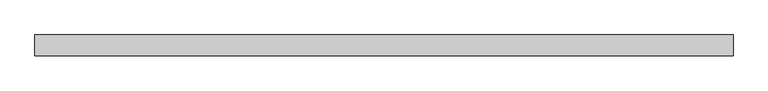
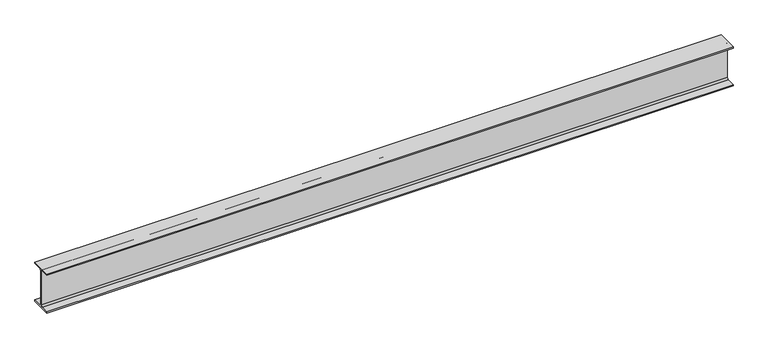
"""IFC4 building model written with IfcOpenShell, lengths in millimetres: beam geometry, 0912_Steel Framing_H-KSD3502 : H_SB_ASB_H-400x200x8x13."""

from ifc_helpers import new_model, si_unit, point, frame, frame_2d, origin, place, context, project, spatial, polyline, circle_curve, trimmed, segment, composite_curve, outline, extrude, source, transform, mapped, element, save


def beam_e35f9711(model_context):
    return source(origin(), model_context, "Body", "SweptSolid", [
        extrude(outline(composite_curve([segment(polyline([(100.0, -187.0), (100.0, -200.0), (-100.0, -200.0), (-100.0, -187.0), (-20.0, -187.0)]), True, "CONTINUOUS"), segment(trimmed(circle_curve(frame_2d((-20.0, -171.0)), 16.0), [point((-20.0, -187.0))], [point((-4.0, -171.0))], True, "CARTESIAN"), True, "CONTINUOUS"), segment(polyline([(-4.0, -171.0), (-4.0, 171.0)]), True, "CONTINUOUS"), segment(trimmed(circle_curve(frame_2d((-20.0, 171.0)), 16.0), [point((-4.0, 171.0))], [point((-20.0, 187.0))], True, "CARTESIAN"), True, "CONTINUOUS"), segment(polyline([(-20.0, 187.0), (-100.0, 187.0), (-100.0, 200.0), (100.0, 200.0), (100.0, 187.0), (20.0, 187.0)]), True, "CONTINUOUS"), segment(trimmed(circle_curve(frame_2d((20.0, 171.0)), 16.0), [point((20.0, 187.0))], [point((4.0, 171.0))], True, "CARTESIAN"), True, "CONTINUOUS"), segment(polyline([(4.0, 171.0), (4.0, -171.0)]), True, "CONTINUOUS"), segment(trimmed(circle_curve(frame_2d((20.0, -171.0)), 16.0), [point((4.0, -171.0))], [point((20.0, -187.0))], True, "CARTESIAN"), True, "CONTINUOUS"), segment(polyline([(20.0, -187.0), (100.0, -187.0)]), True, "CONTINUOUS")], self_intersect=False)), frame((-3244.5360727, 0.0, 0.0), z_axis=(1.0, 0.0, 0.0), x_axis=(0.0, 1.0, 0.0)), (0.0, 0.0, 1.0), 6649.3360727),
    ])


if __name__ == "__main__":
    model = new_model("IFC4")
    model_context = context("Model", 3, world=origin())
    ifc_project = project(units=[si_unit("LENGTHUNIT", "METRE", prefix="MILLI")], contexts=[model_context])
    site = spatial("IfcSite", under=ifc_project)
    building = spatial("IfcBuilding", under=site)
    placement = place(None, origin())
    beam_shape = beam_e35f9711(model_context)
    element("IfcBeam", 1, ObjectType="0912_Steel Framing_H-KSD3502 : H_SB_ASB_H-400x200x8x13", at=placement, inside=building, context=model_context, shape_type="MappedRepresentation", body=[
        mapped(beam_shape, transform((0.0, 0.0, 0.0), x_axis=(1.0, 0.0, 0.0), y_axis=(0.0, 1.0, 0.0), z_axis=(0.0, 0.0, 1.0))),
    ])
    save(model, "model.ifc")

# Revit data of these elements
# Type "0912_Steel Framing_H-KSD3502 : H_SB_ASB_H-400x200x8x13"
#   H_WM Code_1 = "S01AA002-00001 | Main Steel Structure Fabrication Work | Shelter/Building | Medium Steel - Standard (90KG/M>Weight≥30KG/M) | Material: (   )"
#   H_WM Code_2 = "S03AA028-00001 | Main Steel Structure Erection Work | Shelter/Building | Medium Steel (90KG/M>Weight≥30KG/M) | Material: (   )"
#   H_WM Code_3 = "S01AA010-00001 | Main Steel Structure Fabrication Work | Shelter/Building | Steel Painting/Coating | for Non-Fireproofed Steel Surface, Surface Preparation, Primer, Second & Final Coat | Material: (   )"
#   H_Q'ty Cal Type Tag = "SB-Q2"
#   Width = 20.0 cm
#   Web Thickness = 0.8 cm
#   Web Fillet = 1.6 cm
#   Warping Constant = 649000.0 cm⁶
#   W = 0
#   Torsional Moment of Inertia = 35.8981 cm⁴
#   Section Area = 84.12 cm²
#   Plastic Modulus weak axis = 268.0 cm³
#   Plastic Modulus strong axis = 1330.0 cm³
#   Perimeter = 1.56 m²/m
#   Nominal Weight = 66.00 kgf/m
#   Moment of Inertia weak axis = 1740.00 cm⁴
#   Moment of Inertia strong axis = 23700.00 cm⁴
#   Height = 40.0 cm
#   Flange Thickness = 1.3 cm
#   Elastic Modulus weak axis = 174.0 cm³
#   Elastic Modulus strong axis = 1190.0 cm³
#   Centroid Vertical = 20.0 cm
#   Centroid Horizontal = 10.0 cm
#   Ix = 237000000
#   Length [instance default] = 1.5240 m
#   Zx = 1330000
#   b = 0.2000 m
#   h = 0.4000 m
#   r = 0.0160 m
#   s = 0.0080 m
#   t = 0.0130 m
#   A = 0.008412 m²
#   Structural Material [instance default] = Steel, 45-345
#   Assembly Code = ""
# Element 1 (IfcBeam, "0912_Steel Framing_H-KSD3502 : H_SB_ASB_H-400x200x8x13")
#   Structural Material = none
# Materials
#   "Steel, 45-345": class "Metal", colour RGB 189 187 185, transparency 0, Description = "Steel 345 MPa", Cost = 0
